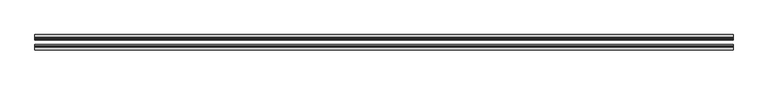
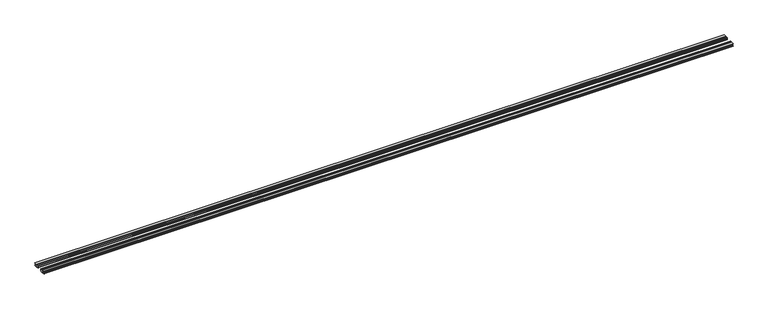
"""IFC4 building model written with IfcOpenShell, lengths in millimetres: proxy geometry, Generic Models 6:Generic Models 2:318829:Generic Models 2:318829 : Generic Models 6:Generic Models 2:318829:7 : Generic Models 6:Generic Models 2:318829:Generic Models 2:318829 : Generic Models 6:Generic Models 2:318829:300683."""

from ifc_helpers import new_model, si_unit, frame, origin, place, context, project, spatial, polyline, outline, extrude, source, transform, mapped, element, save


def generic_models_43baa60a(model_context):
    return source(origin(), model_context, "Body", "SweptSolid", [
        extrude(outline(polyline([(-579041.3240999, 3702.1620698), (-579040.0336784, 3702.7415461), (-579038.0693157, 3704.3667743), (-579037.1687854, 3706.3921459), (-579037.4729673, 3708.5008104), (-579038.9342748, 3710.3628865), (-579041.3240999, 3711.6870698), (-579032.5219617, 3711.6870698), (-579033.0880747, 3710.2384249), (-579033.5586038, 3706.9245698), (-579033.0880747, 3703.6107146), (-579032.5219617, 3702.1620698), (-579041.3240999, 3702.1620698)])), frame((590317.0242239, 0.0, 0.0), z_axis=(1.0, 0.0, 0.0), x_axis=(0.0, 1.0, 0.0)), (0.0, 0.0, 1.0), 2438.4),
        extrude(outline(polyline([(-579046.4591752, 3702.2814756), (-579049.3235965, 3703.2010973), (-579051.3058376, 3704.8581985), (-579052.0132913, 3706.9245698), (-579051.3058376, 3708.9909411), (-579049.3235965, 3710.6480422), (-579046.4591752, 3711.567664), (-579044.8695413, 3711.6870698), (-579043.2799074, 3711.567664), (-579040.415486, 3710.6480422), (-579038.4332449, 3708.9909411), (-579037.7257913, 3706.9245698), (-579038.4332449, 3704.8581985), (-579040.415486, 3703.2010973), (-579043.2799074, 3702.2814756), (-579044.8695413, 3702.1620698), (-579046.4591752, 3702.2814756)])), frame((590317.0242239, 0.0, 0.0), z_axis=(1.0, 0.0, 0.0), x_axis=(0.0, 1.0, 0.0)), (0.0, 0.0, 1.0), 2438.4),
        extrude(outline(polyline([(-579077.5973576, 3702.1620698), (-579086.3994958, 3702.1620698), (-579085.8333829, 3703.6107146), (-579085.3628538, 3706.9245698), (-579085.8333829, 3710.2384249), (-579086.3994958, 3711.6870698), (-579077.5973576, 3711.6870698), (-579079.9871827, 3710.3628865), (-579081.4484902, 3708.5008104), (-579081.7526721, 3706.3921459), (-579080.8521418, 3704.3667743), (-579078.8877791, 3702.7415461), (-579077.5973576, 3702.1620698)])), frame((590317.0242239, 0.0, 0.0), z_axis=(1.0, 0.0, 0.0), x_axis=(0.0, 1.0, 0.0)), (0.0, 0.0, 1.0), 2438.4),
        extrude(outline(polyline([(-579072.4622823, 3702.2814756), (-579074.0519163, 3702.1620698), (-579075.6415502, 3702.2814756), (-579078.5059715, 3703.2010973), (-579080.4882126, 3704.8581985), (-579081.1956663, 3706.9245698), (-579080.4882126, 3708.9909411), (-579078.5059715, 3710.6480422), (-579075.6415502, 3711.567664), (-579074.0519163, 3711.6870698), (-579072.4622823, 3711.567664), (-579069.597861, 3710.6480422), (-579067.6156199, 3708.9909411), (-579066.9081663, 3706.9245698), (-579067.6156199, 3704.8581985), (-579069.597861, 3703.2010973), (-579072.4622823, 3702.2814756)])), frame((590317.0242239, 0.0, 0.0), z_axis=(1.0, 0.0, 0.0), x_axis=(0.0, 1.0, 0.0)), (0.0, 0.0, 1.0), 2438.4),
    ])


if __name__ == "__main__":
    model = new_model("IFC4")
    model_context = context("Model", 3, world=origin())
    ifc_project = project(units=[si_unit("LENGTHUNIT", "METRE", prefix="MILLI")], contexts=[model_context])
    site = spatial("IfcSite", under=ifc_project)
    building = spatial("IfcBuilding", under=site)
    placement = place(None, origin())
    generic_models_shape = generic_models_43baa60a(model_context)
    element("IfcBuildingElementProxy", 1, Name="Generic Models 6:Generic Models 2:318829:Generic Models 2:318829 : Generic Models 6:Generic Models 2:318829:7 : Generic Models 6:Generic Models 2:318829:Generic Models 2:318829 : Generic Models 6:Generic Models 2:318829:300683", ObjectType="Generic Models 6:Generic Models 2:318829:Generic Models 2:318829 : Generic Models 6:Generic Models 2:318829:7 : Generic Models 6:Generic Models 2:318829:Generic Models 2:318829 : Generic Models 6:Generic Models 2:318829:300683", at=placement, inside=building, context=model_context, shape_type="MappedRepresentation", body=[
        mapped(generic_models_shape, transform((0.0, 0.0, 0.0), x_axis=(1.0, 0.0, 0.0), y_axis=(0.0, 1.0, 0.0), z_axis=(0.0, 0.0, 1.0))),
    ])
    save(model, "model.ifc")

# Revit data of these elements
# Type "Generic Models 6:Generic Models 2:318829:Generic Models 2:318829 : Generic Models 6:Generic Models 2:318829:7 : Generic Models 6:Generic Models 2:318829:Generic Models 2:318829 : Generic Models 6:Generic Models 2:318829:300683"
#   NameOverride = "Generic Models 6:Generic Models 2:318829:Generic Models 2:318829 : Generic Models 6:Generic Models 2:318829:300683"
#   ObjectTypeOverride = "Generic Models 2:318829 : Generic Models 6:Generic Models 2:318829"
#   Reference = "Generic Models 2"
#   Tag = "300683"
# Element 1 (IfcBuildingElementProxy, "Generic Models 6:Generic Models 2:318829:Generic Models 2:318829 : Generic Models 6:Generic Models 2:318829:7 : Generic Models 6:Generic Models 2:318829:Generic Models 2:318829 : Generic Models 6:Generic Models 2:318829:300683")
#   Materials on its faces: "SEALANT & BACKER ROD"
# Materials
#   "SEALANT & BACKER ROD": class "Unassigned", colour RGB 120 120 120, transparency 0, Cost = 0
